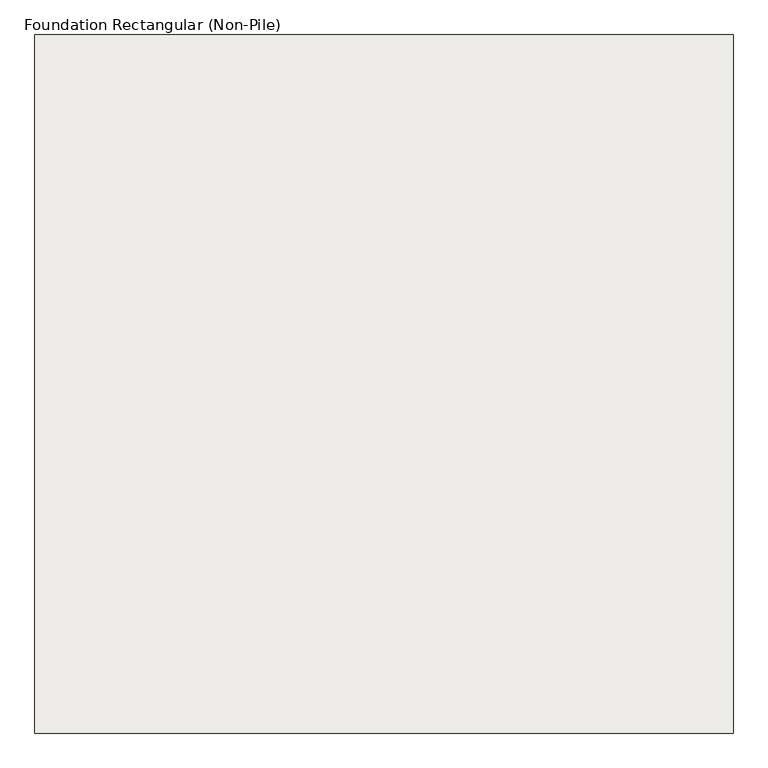
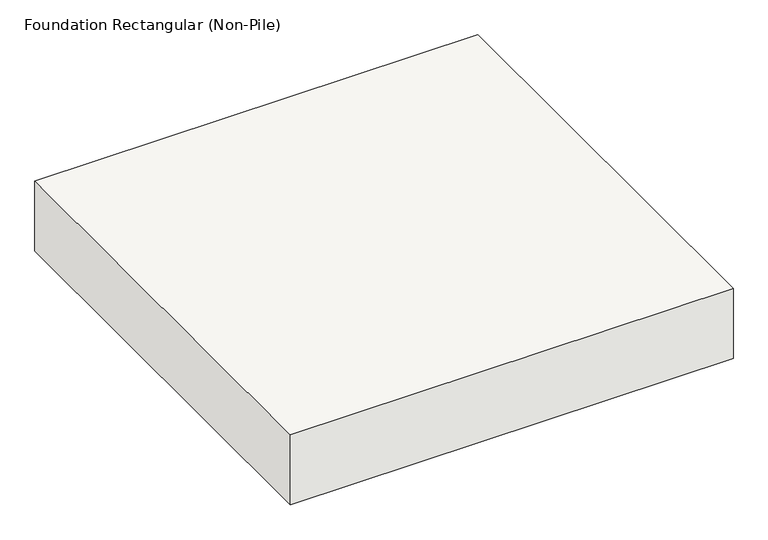
"""IFC4 building model written with IfcOpenShell, lengths in millimetres: slab geometry, Foundation Rectangular (Non-Pile) : H_SF_AR S18_Ret Fdn_F2 3000x3000x500."""

import ifcopenshell
import ifcopenshell.guid

model = None  # the IFC model being written
_history = None  # IfcOwnerHistory: only IFC2X3 demands one
_inside = {}  # id of a spatial element -> (the spatial element, [elements in it])
_under = {}  # id of a project, library or spatial element -> (it, [spatial elements below it])
_declared = {}  # id of a project -> (the project, [libraries it declares])
_typed = {}  # id of a type object -> (the type object, [elements of that type])
_made_of = {}  # id of a material, layer set ... -> (it, [elements and type objects made of it])


def new_model(schema):
    """Start an empty IFC model of exactly this schema.

    Asked for "IFC4X3", IfcOpenShell would pick the latest addendum, in which some entities
    have other attributes; the version numbers below select the first issue.
    IFC2X3 requires an IfcOwnerHistory on every rooted entity: one is made here for all.
    """
    global model, _history
    if schema == "IFC4X3":
        model = ifcopenshell.file(schema_version=(4, 3, 0, 0))
    else:
        model = ifcopenshell.file(schema=schema)
    _inside.clear()
    _under.clear()
    _declared.clear()
    _typed.clear()
    _made_of.clear()
    _history = None
    if model.schema == "IFC2X3":
        org = make("IfcOrganization", Name="unknown")
        user = make(
            "IfcPersonAndOrganization",
            ThePerson=make("IfcPerson", FamilyName="unknown"),
            TheOrganization=org,
        )
        app = make(
            "IfcApplication",
            ApplicationDeveloper=org,
            Version="unknown",
            ApplicationFullName="unknown",
            ApplicationIdentifier="unknown",
        )
        _history = make(
            "IfcOwnerHistory",
            OwningUser=user,
            OwningApplication=app,
            ChangeAction="ADDED",
            CreationDate=0,
        )
    return model


def make(cls, **values):
    """One entity of the class cls with the attributes given. An attribute that is None is left unset."""
    return model.create_entity(
        cls, **{name: value for name, value in values.items() if value is not None}
    )


def rooted(cls, **values):
    """An entity with a GlobalId (a new one), such as an element, a storey or a relation."""
    return make(cls, GlobalId=ifcopenshell.guid.new(), OwnerHistory=_history, **values)


def si_unit(unit_type, name, prefix=None):
    """IfcSIUnit, for example si_unit("LENGTHUNIT", "METRE", prefix="MILLI")."""
    return make("IfcSIUnit", UnitType=unit_type, Prefix=prefix, Name=name)


def assignment(units):
    """IfcUnitAssignment: the units of a project."""
    return None if units is None else make("IfcUnitAssignment", Units=units)


def point(xyz):
    """IfcCartesianPoint."""
    return None if xyz is None else make("IfcCartesianPoint", Coordinates=xyz)


def direction(xyz):
    """IfcDirection."""
    return None if xyz is None else make("IfcDirection", DirectionRatios=xyz)


def frame(location, z_axis=None, x_axis=None):
    """IfcAxis2Placement3D, a coordinate frame: its origin and axes. An axis left out is left unset."""
    return make(
        "IfcAxis2Placement3D",
        Location=point(location),
        Axis=direction(z_axis),
        RefDirection=direction(x_axis),
    )


def origin():
    """The frame at (0, 0, 0) with its axes left unset."""
    return frame((0.0, 0.0, 0.0))


def place(relative_to, where):
    """IfcLocalPlacement: puts the frame where relative to a parent placement (None: the world)."""
    return make(
        "IfcLocalPlacement", PlacementRelTo=relative_to, RelativePlacement=where
    )


def context(
    kind, dimensions, precision=None, world=None, true_north=None, identifier=None
):
    """IfcGeometricRepresentationContext, for example the 3D "Model" context."""
    return make(
        "IfcGeometricRepresentationContext",
        ContextIdentifier=identifier,
        ContextType=kind,
        CoordinateSpaceDimension=dimensions,
        Precision=precision,
        WorldCoordinateSystem=world,
        TrueNorth=true_north,
    )


def project(units=None, contexts=None):
    """IfcProject with its units and contexts."""
    return rooted(
        "IfcProject",
        Name="project",
        RepresentationContexts=contexts,
        UnitsInContext=assignment(units),
    )


def spatial(cls, under=None, at=None, **own):
    """A site, building, storey or space (cls), placed at a placement, below another one or the project."""
    s = rooted(cls, ObjectPlacement=at, **own)
    if under is not None:
        _under.setdefault(under.id(), (under, []))[1].append(s)
    return s


def polyline(points):
    """IfcPolyline through the points."""
    return make("IfcPolyline", Points=[point(p) for p in points])


def outline(outer, holes=None, kind="AREA"):
    """IfcArbitraryClosedProfileDef: a profile drawn as a closed curve; with holes, ...WithVoids."""
    if holes is None:
        return make("IfcArbitraryClosedProfileDef", ProfileType=kind, OuterCurve=outer)
    return make(
        "IfcArbitraryProfileDefWithVoids",
        ProfileType=kind,
        OuterCurve=outer,
        InnerCurves=holes,
    )


def extrude(swept, where, along, depth):
    """IfcExtrudedAreaSolid: the profile swept, set in the frame where, extruded along a direction by depth."""
    return make(
        "IfcExtrudedAreaSolid",
        SweptArea=swept,
        Position=where,
        ExtrudedDirection=direction(along),
        Depth=depth,
    )


def shape(context_of_items, identifier, shape_type, items):
    """IfcShapeRepresentation: the items that make up one representation, for example the "Body"."""
    return make(
        "IfcShapeRepresentation",
        ContextOfItems=context_of_items,
        RepresentationIdentifier=identifier,
        RepresentationType=shape_type,
        Items=items,
    )


def source(mapping_origin, context_of_items, identifier, shape_type, items):
    """IfcRepresentationMap: a shape defined once, which mapped items show again and again."""
    return make(
        "IfcRepresentationMap",
        MappingOrigin=mapping_origin,
        MappedRepresentation=shape(context_of_items, identifier, shape_type, items),
    )


def transform(
    local_origin,
    x_axis=None,
    y_axis=None,
    z_axis=None,
    scale=None,
    scale2=None,
    scale3=None,
    uniform=True,
):
    """IfcCartesianTransformationOperator3D, or its non-uniform kind. x_axis, y_axis, z_axis: its Axis1, 2, 3."""
    if uniform:
        return make(
            "IfcCartesianTransformationOperator3D",
            Axis1=direction(x_axis),
            Axis2=direction(y_axis),
            LocalOrigin=point(local_origin),
            Scale=scale,
            Axis3=direction(z_axis),
        )
    return make(
        "IfcCartesianTransformationOperator3DnonUniform",
        Axis1=direction(x_axis),
        Axis2=direction(y_axis),
        LocalOrigin=point(local_origin),
        Scale=scale,
        Axis3=direction(z_axis),
        Scale2=scale2,
        Scale3=scale3,
    )


def mapped(mapping_source, mapping_target):
    """IfcMappedItem: shows the shape of a source again, moved by a transform."""
    return make(
        "IfcMappedItem", MappingSource=mapping_source, MappingTarget=mapping_target
    )


def made_of(thing, what):
    """Note that an element or type object is made of a material, layer set ...; save() writes the relation."""
    if what is not None:
        _made_of.setdefault(what.id(), (what, []))[1].append(thing)
    return thing


def element(
    cls,
    number,
    at=None,
    inside=None,
    cuts=None,
    type_object=None,
    material=None,
    context=None,
    identifier="Body",
    shape_type=None,
    held_by="IfcProductDefinitionShape",
    body=None,
    shapes=None,
    **own,
):
    """One element of the class cls, such as IfcWall. Its Tag is "e" and its number.

    at: its placement. inside: the storey or other place that contains it. cuts: it is an
    opening in that element (IfcRelVoidsElement). A single representation is given by context,
    identifier, shape_type and body (its items); several are given by shapes. held_by: the class
    of the entity that holds the representations. save() writes the other relations.
    """
    e = rooted(cls, Tag="e%d" % number, ObjectPlacement=at, **own)
    if body is not None:
        shapes = [shape(context, identifier, shape_type, body)]
    if shapes is not None:
        e.Representation = make(held_by, Representations=shapes)
    if inside is not None:
        _inside.setdefault(inside.id(), (inside, []))[1].append(e)
    if cuts is not None:
        rooted(
            "IfcRelVoidsElement", RelatingBuildingElement=cuts, RelatedOpeningElement=e
        )
    if type_object is not None:
        _typed.setdefault(type_object.id(), (type_object, []))[1].append(e)
    return made_of(e, material)


def aggregate(whole, parts):
    """IfcRelAggregates: a whole, such as a stair, and the parts it consists of."""
    return rooted("IfcRelAggregates", RelatingObject=whole, RelatedObjects=parts)


def save(model, path):
    """Write the relations noted so far, then the file.

    IfcRelAggregates (storeys below a building ...), IfcRelContainedInSpatialStructure (elements
    in a storey), IfcRelDefinesByType, IfcRelAssociatesMaterial and IfcRelDeclares: one each for
    every whole, place, type object, material and project.
    """
    for whole, parts in _under.values():
        aggregate(whole, parts)
    for where, things in _inside.values():
        rooted(
            "IfcRelContainedInSpatialStructure",
            RelatedElements=things,
            RelatingStructure=where,
        )
    for kind, things in _typed.values():
        rooted("IfcRelDefinesByType", RelatedObjects=things, RelatingType=kind)
    for what, things in _made_of.values():
        rooted("IfcRelAssociatesMaterial", RelatedObjects=things, RelatingMaterial=what)
    for by, libraries in _declared.values():
        rooted("IfcRelDeclares", RelatingContext=by, RelatedDefinitions=libraries)
    model.write(path)


def foundation_rectangular_non_pile_a43cc813(model_context):
    return source(origin(), model_context, "Body", "SweptSolid", [
        extrude(outline(polyline([(1500.0, 1500.0), (1500.0, -1500.0), (-1500.0, -1500.0), (-1500.0, 1500.0), (1500.0, 1500.0)])), frame((0.0, 0.0, -500.0), z_axis=(0.0, 0.0, 1.0), x_axis=(1.0, 0.0, 0.0)), (0.0, 0.0, 1.0), 500.0),
    ])


if __name__ == "__main__":
    model = new_model("IFC4")
    model_context = context("Model", 3, world=origin())
    ifc_project = project(units=[si_unit("LENGTHUNIT", "METRE", prefix="MILLI")], contexts=[model_context])
    site = spatial("IfcSite", under=ifc_project)
    building = spatial("IfcBuilding", under=site)
    placement = place(None, origin())
    foundation_rectangular_non_pile_shape = foundation_rectangular_non_pile_a43cc813(model_context)
    element("IfcSlab", 1, ObjectType="Foundation Rectangular (Non-Pile) : H_SF_AR S18_Ret Fdn_F2 3000x3000x500", at=placement, inside=building, context=model_context, shape_type="MappedRepresentation", body=[
        mapped(foundation_rectangular_non_pile_shape, transform((0.0, 0.0, 0.0), x_axis=(1.0, 0.0, 0.0), y_axis=(0.0, 1.0, 0.0), z_axis=(0.0, 0.0, 1.0))),
    ])
    save(model, "model.ifc")

# Revit data of these elements
# Type "Foundation Rectangular (Non-Pile) : H_SF_AR S18_Ret Fdn_F2 3000x3000x500"
#   Type Comments = "UG"
#   Type Mark = "F2"
#   Top bar = "D25@300"
#   Description = "UG Shallow Foundation"
#   Bottom bar = "D20@300"
#   H_Rebar Ratio = 0.12
#   Width = 3000 mm
#   Length = 3000 mm
#   Foundation Thickness = 500 mm
#   Structural Material [instance default] = none
#   Assembly Code = ""
# Element 1 (IfcSlab, "Foundation Rectangular (Non-Pile) : H_SF_AR S18_Ret Fdn_F2 3000x3000x500")
#   Materials on its faces: "00_Concrete_Reinf. Conc."
# Materials
#   "00_Concrete_Reinf. Conc.": class "Concrete", colour RGB 176 176 176, transparency 0, Description = "Reinf. Conc.", Cost = 0, Image = Concrete.Cast-In-Place.Flat.Polished.Grey.jpg
